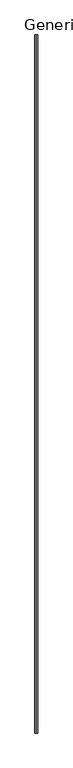
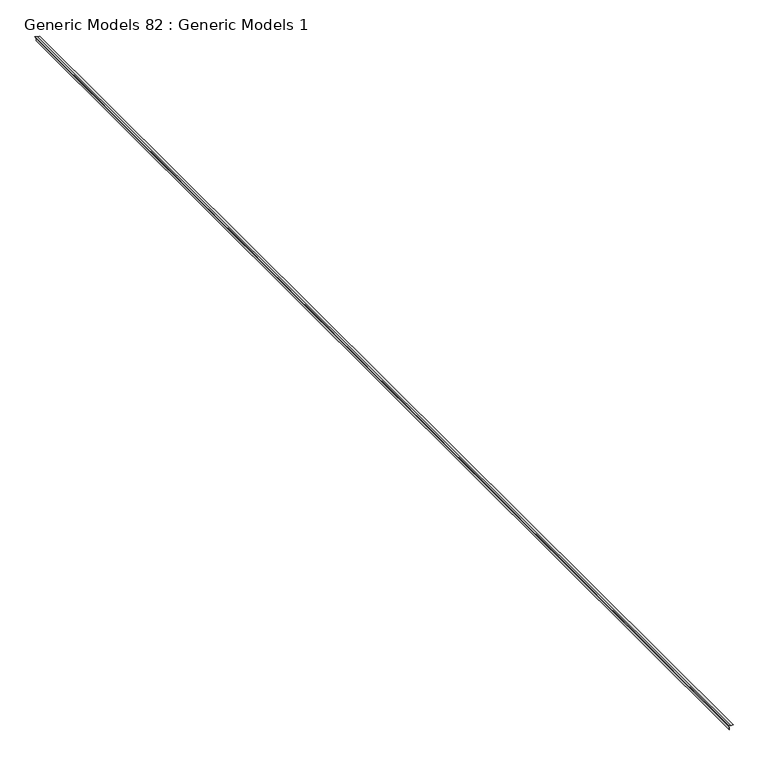
"""IFC4 building model written with IfcOpenShell, lengths in millimetres: proxy geometry, Generic Models 82 : Generic Models 1."""

from ifc_helpers import new_model, si_unit, point, frame, frame_2d, origin, place, context, project, spatial, polyline, circle_curve, trimmed, segment, composite_curve, outline, extrude, source, transform, mapped, element, save


def generic_models_82_generic_models_1_3673b194(model_context):
    return source(origin(), model_context, "Body", "SweptSolid", [
        extrude(outline(composite_curve([segment(trimmed(circle_curve(frame_2d((127127.2167873, 9448.0457008)), 1.4342127), [point((127128.4926156, 9448.7008558))], [point((127126.5616323, 9446.7698725))], False, "CARTESIAN"), True, "CONTINUOUS"), segment(polyline([(127126.5616323, 9446.7698725), (127088.5361176, 9466.2964881), (127050.4361176, 9466.2964881), (127050.4361176, 9467.5664881), (127088.8431414, 9467.5664881), (127127.5962396, 9447.6662484), (127107.696, 9486.4193467), (127107.696, 9524.8263704), (127108.966, 9524.8263704), (127108.966, 9486.7263704), (127128.4926156, 9448.7008558)]), True, "CONTINUOUS")], self_intersect=False)), frame((0.0, -7068.1230338, 0.0), z_axis=(0.0, 1.0, 0.0), x_axis=(0.0, 0.0, 1.0)), (0.0, 0.0, 1.0), 19050.0),
    ])


if __name__ == "__main__":
    model = new_model("IFC4")
    model_context = context("Model", 3, world=origin())
    ifc_project = project(units=[si_unit("LENGTHUNIT", "METRE", prefix="MILLI")], contexts=[model_context])
    site = spatial("IfcSite", under=ifc_project)
    building = spatial("IfcBuilding", under=site)
    placement = place(None, origin())
    generic_models_82_generic_models_1_shape = generic_models_82_generic_models_1_3673b194(model_context)
    element("IfcBuildingElementProxy", 1, Name="Generic Models 82 : Generic Models 1", ObjectType="Generic Models 82 : Generic Models 1", at=placement, inside=building, context=model_context, shape_type="MappedRepresentation", body=[
        mapped(generic_models_82_generic_models_1_shape, transform((0.0, 0.0, 0.0), x_axis=(1.0, 0.0, 0.0), y_axis=(0.0, 1.0, 0.0), z_axis=(0.0, 0.0, 1.0))),
    ])
    save(model, "model.ifc")

# Revit data of these elements
# Element 1 (IfcBuildingElementProxy, "Generic Models 82 : Generic Models 1")
#   Materials on its faces: "_CONTINUOUS 16 GA. COPPER CORNER BEAD"
# Materials
#   "_CONTINUOUS 16 GA. COPPER CORNER BEAD": class "Generic", colour RGB 253 192 103, transparency 0, Cost = 0
